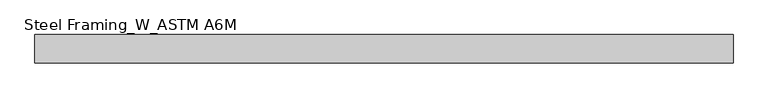
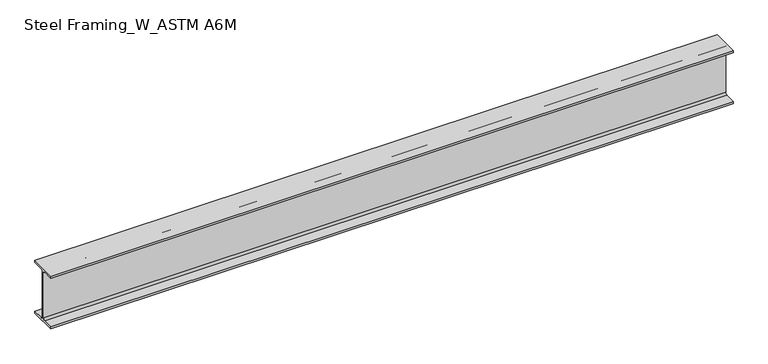
"""IFC4 building model written with IfcOpenShell, lengths in millimetres: beam geometry, Steel Framing_W_ASTM A6M : H_SB_AR_S02_W200x22.5_J1."""

import ifcopenshell
import ifcopenshell.guid

model = None  # the IFC model being written
_history = None  # IfcOwnerHistory: only IFC2X3 demands one
_inside = {}  # id of a spatial element -> (the spatial element, [elements in it])
_under = {}  # id of a project, library or spatial element -> (it, [spatial elements below it])
_declared = {}  # id of a project -> (the project, [libraries it declares])
_typed = {}  # id of a type object -> (the type object, [elements of that type])
_made_of = {}  # id of a material, layer set ... -> (it, [elements and type objects made of it])


def new_model(schema):
    """Start an empty IFC model of exactly this schema.

    Asked for "IFC4X3", IfcOpenShell would pick the latest addendum, in which some entities
    have other attributes; the version numbers below select the first issue.
    IFC2X3 requires an IfcOwnerHistory on every rooted entity: one is made here for all.
    """
    global model, _history
    if schema == "IFC4X3":
        model = ifcopenshell.file(schema_version=(4, 3, 0, 0))
    else:
        model = ifcopenshell.file(schema=schema)
    _inside.clear()
    _under.clear()
    _declared.clear()
    _typed.clear()
    _made_of.clear()
    _history = None
    if model.schema == "IFC2X3":
        org = make("IfcOrganization", Name="unknown")
        user = make(
            "IfcPersonAndOrganization",
            ThePerson=make("IfcPerson", FamilyName="unknown"),
            TheOrganization=org,
        )
        app = make(
            "IfcApplication",
            ApplicationDeveloper=org,
            Version="unknown",
            ApplicationFullName="unknown",
            ApplicationIdentifier="unknown",
        )
        _history = make(
            "IfcOwnerHistory",
            OwningUser=user,
            OwningApplication=app,
            ChangeAction="ADDED",
            CreationDate=0,
        )
    return model


def make(cls, **values):
    """One entity of the class cls with the attributes given. An attribute that is None is left unset."""
    return model.create_entity(
        cls, **{name: value for name, value in values.items() if value is not None}
    )


def rooted(cls, **values):
    """An entity with a GlobalId (a new one), such as an element, a storey or a relation."""
    return make(cls, GlobalId=ifcopenshell.guid.new(), OwnerHistory=_history, **values)


def si_unit(unit_type, name, prefix=None):
    """IfcSIUnit, for example si_unit("LENGTHUNIT", "METRE", prefix="MILLI")."""
    return make("IfcSIUnit", UnitType=unit_type, Prefix=prefix, Name=name)


def assignment(units):
    """IfcUnitAssignment: the units of a project."""
    return None if units is None else make("IfcUnitAssignment", Units=units)


def point(xyz):
    """IfcCartesianPoint."""
    return None if xyz is None else make("IfcCartesianPoint", Coordinates=xyz)


def direction(xyz):
    """IfcDirection."""
    return None if xyz is None else make("IfcDirection", DirectionRatios=xyz)


def frame(location, z_axis=None, x_axis=None):
    """IfcAxis2Placement3D, a coordinate frame: its origin and axes. An axis left out is left unset."""
    return make(
        "IfcAxis2Placement3D",
        Location=point(location),
        Axis=direction(z_axis),
        RefDirection=direction(x_axis),
    )


def frame_2d(location, x_axis=None):
    """IfcAxis2Placement2D, a coordinate frame in the plane: its origin and x axis."""
    return make(
        "IfcAxis2Placement2D", Location=point(location), RefDirection=direction(x_axis)
    )


def origin():
    """The frame at (0, 0, 0) with its axes left unset."""
    return frame((0.0, 0.0, 0.0))


def place(relative_to, where):
    """IfcLocalPlacement: puts the frame where relative to a parent placement (None: the world)."""
    return make(
        "IfcLocalPlacement", PlacementRelTo=relative_to, RelativePlacement=where
    )


def context(
    kind, dimensions, precision=None, world=None, true_north=None, identifier=None
):
    """IfcGeometricRepresentationContext, for example the 3D "Model" context."""
    return make(
        "IfcGeometricRepresentationContext",
        ContextIdentifier=identifier,
        ContextType=kind,
        CoordinateSpaceDimension=dimensions,
        Precision=precision,
        WorldCoordinateSystem=world,
        TrueNorth=true_north,
    )


def project(units=None, contexts=None):
    """IfcProject with its units and contexts."""
    return rooted(
        "IfcProject",
        Name="project",
        RepresentationContexts=contexts,
        UnitsInContext=assignment(units),
    )


def spatial(cls, under=None, at=None, **own):
    """A site, building, storey or space (cls), placed at a placement, below another one or the project."""
    s = rooted(cls, ObjectPlacement=at, **own)
    if under is not None:
        _under.setdefault(under.id(), (under, []))[1].append(s)
    return s


def polyline(points):
    """IfcPolyline through the points."""
    return make("IfcPolyline", Points=[point(p) for p in points])


def circle_curve(where, radius):
    """IfcCircle in the frame where."""
    return make("IfcCircle", Position=where, Radius=radius)


def trimmed(basis, trim1, trim2, sense, master):
    """IfcTrimmedCurve: the piece of a basis curve between two trims."""
    return make(
        "IfcTrimmedCurve",
        BasisCurve=basis,
        Trim1=trim1,
        Trim2=trim2,
        SenseAgreement=sense,
        MasterRepresentation=master,
    )


def segment(curve, same_sense, transition):
    """IfcCompositeCurveSegment."""
    return make(
        "IfcCompositeCurveSegment",
        Transition=transition,
        SameSense=same_sense,
        ParentCurve=curve,
    )


def composite_curve(segments, self_intersect=None):
    """IfcCompositeCurve: segments joined end to end."""
    return make("IfcCompositeCurve", Segments=segments, SelfIntersect=self_intersect)


def outline(outer, holes=None, kind="AREA"):
    """IfcArbitraryClosedProfileDef: a profile drawn as a closed curve; with holes, ...WithVoids."""
    if holes is None:
        return make("IfcArbitraryClosedProfileDef", ProfileType=kind, OuterCurve=outer)
    return make(
        "IfcArbitraryProfileDefWithVoids",
        ProfileType=kind,
        OuterCurve=outer,
        InnerCurves=holes,
    )


def extrude(swept, where, along, depth):
    """IfcExtrudedAreaSolid: the profile swept, set in the frame where, extruded along a direction by depth."""
    return make(
        "IfcExtrudedAreaSolid",
        SweptArea=swept,
        Position=where,
        ExtrudedDirection=direction(along),
        Depth=depth,
    )


def shape(context_of_items, identifier, shape_type, items):
    """IfcShapeRepresentation: the items that make up one representation, for example the "Body"."""
    return make(
        "IfcShapeRepresentation",
        ContextOfItems=context_of_items,
        RepresentationIdentifier=identifier,
        RepresentationType=shape_type,
        Items=items,
    )


def source(mapping_origin, context_of_items, identifier, shape_type, items):
    """IfcRepresentationMap: a shape defined once, which mapped items show again and again."""
    return make(
        "IfcRepresentationMap",
        MappingOrigin=mapping_origin,
        MappedRepresentation=shape(context_of_items, identifier, shape_type, items),
    )


def transform(
    local_origin,
    x_axis=None,
    y_axis=None,
    z_axis=None,
    scale=None,
    scale2=None,
    scale3=None,
    uniform=True,
):
    """IfcCartesianTransformationOperator3D, or its non-uniform kind. x_axis, y_axis, z_axis: its Axis1, 2, 3."""
    if uniform:
        return make(
            "IfcCartesianTransformationOperator3D",
            Axis1=direction(x_axis),
            Axis2=direction(y_axis),
            LocalOrigin=point(local_origin),
            Scale=scale,
            Axis3=direction(z_axis),
        )
    return make(
        "IfcCartesianTransformationOperator3DnonUniform",
        Axis1=direction(x_axis),
        Axis2=direction(y_axis),
        LocalOrigin=point(local_origin),
        Scale=scale,
        Axis3=direction(z_axis),
        Scale2=scale2,
        Scale3=scale3,
    )


def mapped(mapping_source, mapping_target):
    """IfcMappedItem: shows the shape of a source again, moved by a transform."""
    return make(
        "IfcMappedItem", MappingSource=mapping_source, MappingTarget=mapping_target
    )


def made_of(thing, what):
    """Note that an element or type object is made of a material, layer set ...; save() writes the relation."""
    if what is not None:
        _made_of.setdefault(what.id(), (what, []))[1].append(thing)
    return thing


def element(
    cls,
    number,
    at=None,
    inside=None,
    cuts=None,
    type_object=None,
    material=None,
    context=None,
    identifier="Body",
    shape_type=None,
    held_by="IfcProductDefinitionShape",
    body=None,
    shapes=None,
    **own,
):
    """One element of the class cls, such as IfcWall. Its Tag is "e" and its number.

    at: its placement. inside: the storey or other place that contains it. cuts: it is an
    opening in that element (IfcRelVoidsElement). A single representation is given by context,
    identifier, shape_type and body (its items); several are given by shapes. held_by: the class
    of the entity that holds the representations. save() writes the other relations.
    """
    e = rooted(cls, Tag="e%d" % number, ObjectPlacement=at, **own)
    if body is not None:
        shapes = [shape(context, identifier, shape_type, body)]
    if shapes is not None:
        e.Representation = make(held_by, Representations=shapes)
    if inside is not None:
        _inside.setdefault(inside.id(), (inside, []))[1].append(e)
    if cuts is not None:
        rooted(
            "IfcRelVoidsElement", RelatingBuildingElement=cuts, RelatedOpeningElement=e
        )
    if type_object is not None:
        _typed.setdefault(type_object.id(), (type_object, []))[1].append(e)
    return made_of(e, material)


def aggregate(whole, parts):
    """IfcRelAggregates: a whole, such as a stair, and the parts it consists of."""
    return rooted("IfcRelAggregates", RelatingObject=whole, RelatedObjects=parts)


def save(model, path):
    """Write the relations noted so far, then the file.

    IfcRelAggregates (storeys below a building ...), IfcRelContainedInSpatialStructure (elements
    in a storey), IfcRelDefinesByType, IfcRelAssociatesMaterial and IfcRelDeclares: one each for
    every whole, place, type object, material and project.
    """
    for whole, parts in _under.values():
        aggregate(whole, parts)
    for where, things in _inside.values():
        rooted(
            "IfcRelContainedInSpatialStructure",
            RelatedElements=things,
            RelatingStructure=where,
        )
    for kind, things in _typed.values():
        rooted("IfcRelDefinesByType", RelatedObjects=things, RelatingType=kind)
    for what, things in _made_of.values():
        rooted("IfcRelAssociatesMaterial", RelatedObjects=things, RelatingMaterial=what)
    for by, libraries in _declared.values():
        rooted("IfcRelDeclares", RelatingContext=by, RelatedDefinitions=libraries)
    model.write(path)


def steel_framing_w_astm_a6m_0cfad42d(model_context):
    return source(origin(), model_context, "Body", "SweptSolid", [
        extrude(outline(composite_curve([segment(polyline([(51.0, -95.0), (51.0, -103.0), (-51.0, -103.0), (-51.0, -95.0), (-10.71, -95.0)]), True, "CONTINUOUS"), segment(trimmed(circle_curve(frame_2d((-10.71, -87.4)), 7.6), [point((-10.71, -95.0))], [point((-3.11, -87.4))], True, "CARTESIAN"), True, "CONTINUOUS"), segment(polyline([(-3.11, -87.4), (-3.11, 87.4)]), True, "CONTINUOUS"), segment(trimmed(circle_curve(frame_2d((-10.71, 87.4)), 7.6), [point((-3.11, 87.4))], [point((-10.71, 95.0))], True, "CARTESIAN"), True, "CONTINUOUS"), segment(polyline([(-10.71, 95.0), (-51.0, 95.0), (-51.0, 103.0), (51.0, 103.0), (51.0, 95.0), (10.71, 95.0)]), True, "CONTINUOUS"), segment(trimmed(circle_curve(frame_2d((10.71, 87.4)), 7.6), [point((10.71, 95.0))], [point((3.11, 87.4))], True, "CARTESIAN"), True, "CONTINUOUS"), segment(polyline([(3.11, 87.4), (3.11, -87.4)]), True, "CONTINUOUS"), segment(trimmed(circle_curve(frame_2d((10.71, -87.4)), 7.6), [point((3.11, -87.4))], [point((10.71, -95.0))], True, "CARTESIAN"), True, "CONTINUOUS"), segment(polyline([(10.71, -95.0), (51.0, -95.0)]), True, "CONTINUOUS")], self_intersect=False)), frame((-1195.3, 0.0, 0.0), z_axis=(1.0, 0.0, 0.0), x_axis=(0.0, 1.0, 0.0)), (0.0, 0.0, 1.0), 2517.5),
    ])


if __name__ == "__main__":
    model = new_model("IFC4")
    model_context = context("Model", 3, world=origin())
    ifc_project = project(units=[si_unit("LENGTHUNIT", "METRE", prefix="MILLI")], contexts=[model_context])
    site = spatial("IfcSite", under=ifc_project)
    building = spatial("IfcBuilding", under=site)
    placement = place(None, origin())
    steel_framing_w_astm_a6m_shape = steel_framing_w_astm_a6m_0cfad42d(model_context)
    element("IfcBeam", 1, ObjectType="Steel Framing_W_ASTM A6M : H_SB_AR_S02_W200x22.5_J1", at=placement, inside=building, context=model_context, shape_type="MappedRepresentation", body=[
        mapped(steel_framing_w_astm_a6m_shape, transform((0.0, 0.0, 0.0), x_axis=(1.0, 0.0, 0.0), y_axis=(0.0, 1.0, 0.0), z_axis=(0.0, 0.0, 1.0))),
    ])
    save(model, "model.ifc")

# Revit data of these elements
# Type "Steel Framing_W_ASTM A6M : H_SB_AR_S02_W200x22.5_J1"
#   Section Name Key = "W8x15"
#   Width = 10.2 cm
#   Web Thickness = 0.622 cm
#   Web Fillet = 0.76 cm
#   Warping Constant = 13900.0 cm⁶
#   Torsional Moment of Inertia = 5.70 cm⁴
#   Section Area = 28.6 cm²
#   Plastic Modulus weak axis = 43.8 cm³
#   Plastic Modulus strong axis = 223.0 cm³
#   Perimeter = 0.795 m²/m
#   Nominal Weight = 22.50 kgf/m
#   Moment of Inertia weak axis = 142.00 cm⁴
#   Moment of Inertia strong axis = 2000.00 cm⁴
#   Height = 20.6 cm
#   Flange Thickness = 0.8 cm
#   Elastic Modulus weak axis = 27.9 cm³
#   Elastic Modulus strong axis = 193.0 cm³
#   Centroid Vertical = 10.3 cm
#   Centroid Horizontal = 5.1 cm
#   Length [instance default] = 1500 mm
#   Structural Material [instance default] = Steel, 45-345
#   Bolt Spacing = 0
#   Assembly Code = ""
# Element 1 (IfcBeam, "Steel Framing_W_ASTM A6M : H_SB_AR_S02_W200x22.5_J1")
#   Materials on its faces: "Steel, 45-345"
# Materials
#   "Steel, 45-345": class "Metal", colour RGB 189 187 185, transparency 0, Description = "Steel 345 MPa", Cost = 0
